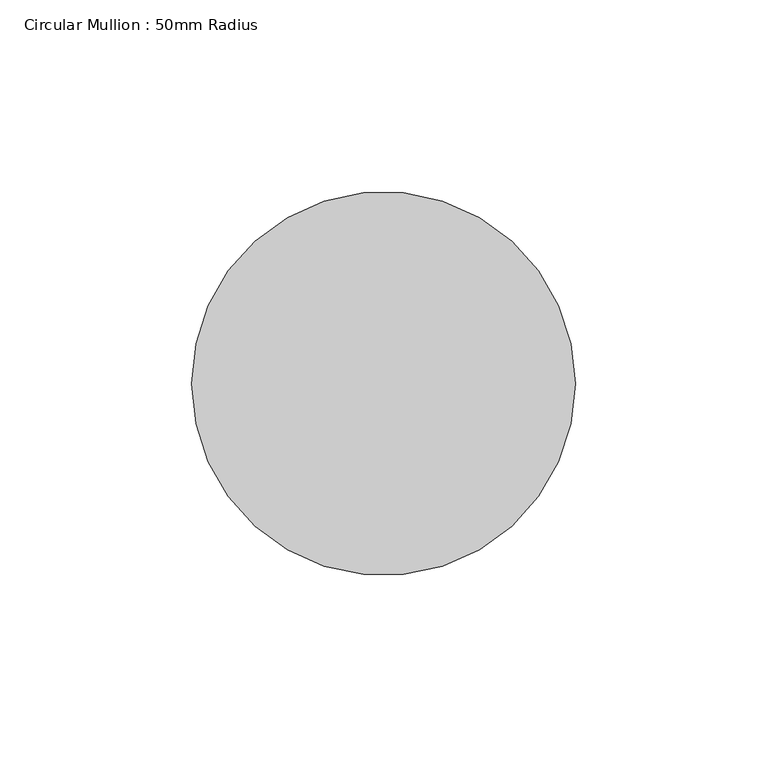
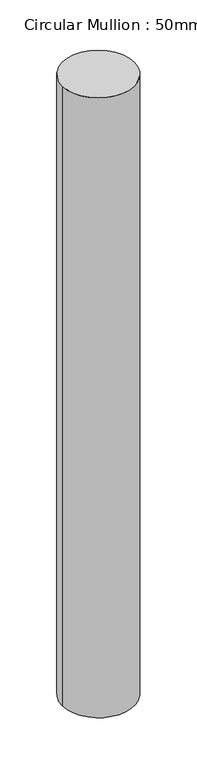
"""IFC4 building model written with IfcOpenShell, lengths in millimetres: member geometry, Circular Mullion : 50mm Radius."""

from ifc_helpers import new_model, si_unit, point, frame, origin, origin_2d, place, context, project, spatial, circle_curve, trimmed, segment, composite_curve, outline, extrude, source, transform, mapped, element, save


def circular_mullion_50mm_radius_21289221(model_context):
    return source(origin(), model_context, "Body", "SweptSolid", [
        extrude(outline(composite_curve([segment(trimmed(circle_curve(origin_2d(), 50.0), [point((50.0, 0.0))], [point((-50.0, 0.0))], False, "CARTESIAN"), True, "CONTINUOUS"), segment(trimmed(circle_curve(origin_2d(), 50.0), [point((-50.0, 0.0))], [point((50.0, 0.0))], False, "CARTESIAN"), True, "CONTINUOUS")], self_intersect=False)), frame((0.0, 0.0, -910.0639454), z_axis=(0.0, 0.0, 1.0), x_axis=(1.0, 0.0, 0.0)), (0.0, 0.0, 1.0), 910.0639454),
    ])


if __name__ == "__main__":
    model = new_model("IFC4")
    model_context = context("Model", 3, world=origin())
    ifc_project = project(units=[si_unit("LENGTHUNIT", "METRE", prefix="MILLI")], contexts=[model_context])
    site = spatial("IfcSite", under=ifc_project)
    building = spatial("IfcBuilding", under=site)
    placement = place(None, origin())
    circular_mullion_50mm_radius_shape = circular_mullion_50mm_radius_21289221(model_context)
    element("IfcMember", 1, ObjectType="Circular Mullion : 50mm Radius", at=placement, inside=building, context=model_context, shape_type="MappedRepresentation", body=[
        mapped(circular_mullion_50mm_radius_shape, transform((0.0, 0.0, 0.0), x_axis=(1.0, 0.0, 0.0), y_axis=(0.0, 1.0, 0.0), z_axis=(0.0, 0.0, 1.0))),
    ])
    save(model, "model.ifc")

# Revit data of these elements
# Type "Circular Mullion : 50mm Radius"
#   built-in parameter 1007350 = 0.164042 (stored number, unit not read)
# Element 1 (IfcMember, "Circular Mullion : 50mm Radius")
#   Materials on its faces: "Aluminium"
# Materials
#   "Aluminium": class "Metal", colour RGB 247 247 247, transparency 0, Description = "Aluminium 6061", Cost = 0
